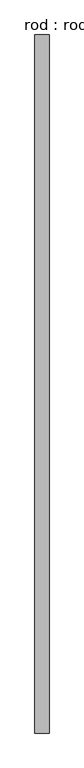
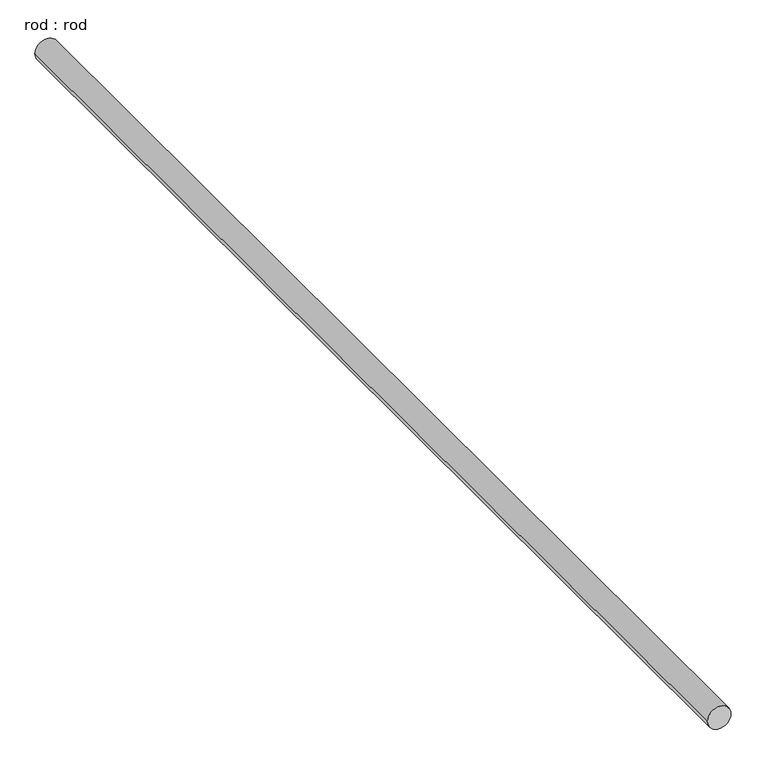
"""IFC4 building model written with IfcOpenShell, lengths in millimetres: proxy geometry, rod : rod."""

from ifc_helpers import new_model, si_unit, point, frame, frame_2d, origin, place, context, project, spatial, circle_curve, trimmed, segment, composite_curve, outline, extrude, source, transform, mapped, element, save


def rod_rod_1a72288e(model_context):
    return source(origin(), model_context, "Body", "SweptSolid", [
        extrude(outline(composite_curve([segment(trimmed(circle_curve(frame_2d((0.0108462, 0.0)), 200.0), [point((0.0108462, 200.0))], [point((0.0108462, -200.0))], False, "CARTESIAN"), True, "CONTINUOUS"), segment(trimmed(circle_curve(frame_2d((0.0108462, 0.0)), 200.0), [point((0.0108462, -200.0))], [point((0.0108462, 200.0))], False, "CARTESIAN"), True, "CONTINUOUS")], self_intersect=False)), frame((0.0, -5794.2819741, 0.0), z_axis=(0.0, 1.0, 0.0), x_axis=(0.0, 0.0, 1.0)), (0.0, 0.0, 1.0), 19774.0211788),
    ])


if __name__ == "__main__":
    model = new_model("IFC4")
    model_context = context("Model", 3, world=origin())
    ifc_project = project(units=[si_unit("LENGTHUNIT", "METRE", prefix="MILLI")], contexts=[model_context])
    site = spatial("IfcSite", under=ifc_project)
    building = spatial("IfcBuilding", under=site)
    placement = place(None, origin())
    rod_rod_shape = rod_rod_1a72288e(model_context)
    element("IfcBuildingElementProxy", 1, Name="rod : rod", ObjectType="rod : rod", at=placement, inside=building, context=model_context, shape_type="MappedRepresentation", body=[
        mapped(rod_rod_shape, transform((0.0, 0.0, 0.0), x_axis=(1.0, 0.0, 0.0), y_axis=(0.0, 1.0, 0.0), z_axis=(0.0, 0.0, 1.0))),
    ])
    save(model, "model.ifc")

# Revit data of these elements
# Type "rod : rod"
#   Default Elevation = 0
